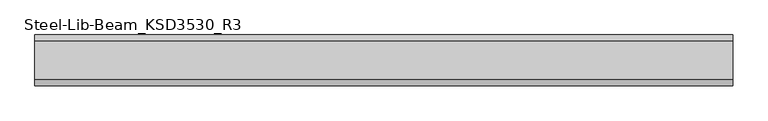
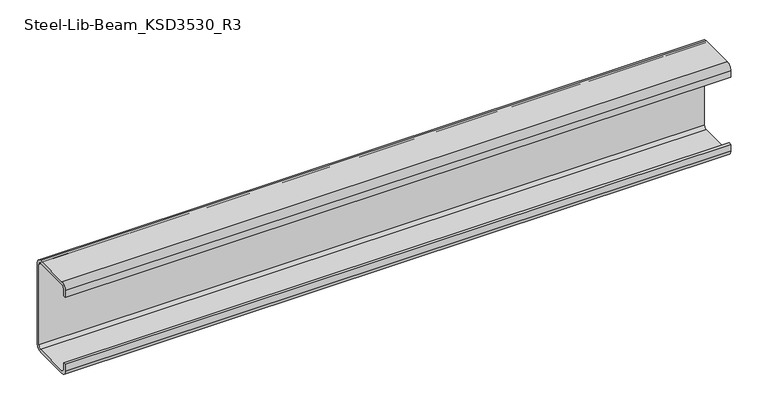
"""IFC4 building model written with IfcOpenShell, lengths in millimetres: beam geometry, Steel-Lib-Beam_KSD3530_R3 : BMS291_C-150×75x20x4.5."""

from ifc_helpers import new_model, si_unit, point, frame, frame_2d, origin, place, context, project, spatial, polyline, circle_curve, trimmed, segment, composite_curve, outline, extrude, source, transform, mapped, element, save


def steel_lib_beam_ksd3530_r3_d74f8c38(model_context):
    return source(origin(), model_context, "Body", "SweptSolid", [
        extrude(outline(composite_curve([segment(trimmed(circle_curve(frame_2d((-41.0, 66.0)), 9.0), [point((-50.0, 66.0))], [point((-41.0, 75.0))], False, "CARTESIAN"), True, "CONTINUOUS"), segment(polyline([(-41.0, 75.0), (16.0, 75.0)]), True, "CONTINUOUS"), segment(trimmed(circle_curve(frame_2d((16.0, 66.0)), 9.0), [point((16.0, 75.0))], [point((25.0, 66.0))], False, "CARTESIAN"), True, "CONTINUOUS"), segment(polyline([(25.0, 66.0), (25.0, -66.0)]), True, "CONTINUOUS"), segment(trimmed(circle_curve(frame_2d((16.0, -66.0)), 9.0), [point((25.0, -66.0))], [point((16.0, -75.0))], False, "CARTESIAN"), True, "CONTINUOUS"), segment(polyline([(16.0, -75.0), (-41.0, -75.0)]), True, "CONTINUOUS"), segment(trimmed(circle_curve(frame_2d((-41.0, -66.0)), 9.0), [point((-41.0, -75.0))], [point((-50.0, -66.0))], False, "CARTESIAN"), True, "CONTINUOUS"), segment(polyline([(-50.0, -66.0), (-50.0, -55.0), (-45.5, -55.0), (-45.5, -66.0)]), True, "CONTINUOUS"), segment(trimmed(circle_curve(frame_2d((-41.0, -66.0)), 4.5), [point((-45.5, -66.0))], [point((-41.0, -70.5))], True, "CARTESIAN"), True, "CONTINUOUS"), segment(polyline([(-41.0, -70.5), (16.0, -70.5)]), True, "CONTINUOUS"), segment(trimmed(circle_curve(frame_2d((16.0, -66.0)), 4.5), [point((16.0, -70.5))], [point((20.5, -66.0))], True, "CARTESIAN"), True, "CONTINUOUS"), segment(polyline([(20.5, -66.0), (20.5, 66.0)]), True, "CONTINUOUS"), segment(trimmed(circle_curve(frame_2d((16.0, 66.0)), 4.5), [point((20.5, 66.0))], [point((16.0, 70.5))], True, "CARTESIAN"), True, "CONTINUOUS"), segment(polyline([(16.0, 70.5), (-41.0, 70.5)]), True, "CONTINUOUS"), segment(trimmed(circle_curve(frame_2d((-41.0, 66.0)), 4.5), [point((-41.0, 70.5))], [point((-45.5, 66.0))], True, "CARTESIAN"), True, "CONTINUOUS"), segment(polyline([(-45.5, 66.0), (-45.5, 55.0), (-50.0, 55.0), (-50.0, 66.0)]), True, "CONTINUOUS")], self_intersect=False)), frame((-515.0, 0.0, 0.0), z_axis=(1.0, 0.0, 0.0), x_axis=(0.0, 1.0, 0.0)), (0.0, 0.0, 1.0), 1030.0),
    ])


if __name__ == "__main__":
    model = new_model("IFC4")
    model_context = context("Model", 3, world=origin())
    ifc_project = project(units=[si_unit("LENGTHUNIT", "METRE", prefix="MILLI")], contexts=[model_context])
    site = spatial("IfcSite", under=ifc_project)
    building = spatial("IfcBuilding", under=site)
    placement = place(None, origin())
    steel_lib_beam_ksd3530_r3_shape = steel_lib_beam_ksd3530_r3_d74f8c38(model_context)
    element("IfcBeam", 1, ObjectType="Steel-Lib-Beam_KSD3530_R3 : BMS291_C-150×75x20x4.5", at=placement, inside=building, context=model_context, shape_type="MappedRepresentation", body=[
        mapped(steel_lib_beam_ksd3530_r3_shape, transform((0.0, 0.0, 0.0), x_axis=(1.0, 0.0, 0.0), y_axis=(0.0, 1.0, 0.0), z_axis=(0.0, 0.0, 1.0))),
    ])
    save(model, "model.ifc")

# Revit data of these elements
# Type "Steel-Lib-Beam_KSD3530_R3 : BMS291_C-150×75x20x4.5"
#   Keynote = "C-150×75x20x4.5"
#   SteelWeight = "Light"
#   x = 0.0250 m
#   t1 = 0.0090 m
#   t = 0.0045 m
#   Surface Area = 0.629834 m²/m
#   Section Area = 13.9688 cm²
#   Mass per Unit Length = 10.9655 kg/m
#   C = 0.0200 m
#   A = 0.0750 m
#   Length [instance default] = 1.5000 m
#   H = 0.1500 m
#   hec_material4 [instance default] = none
#   hec_material3 [instance default] = none
#   hec_material2 [instance default] = none
#   hec_material1 [instance default] = none
#   Structural Material [instance default] = Metal - Steel - Light Gauge
#   Assembly Code = ""
# Element 1 (IfcBeam, "Steel-Lib-Beam_KSD3530_R3 : BMS291_C-150×75x20x4.5")
#   Structural Material = none
# Materials
#   "Metal - Steel - Light Gauge": class "Metal", colour RGB 247 247 247, transparency 0
